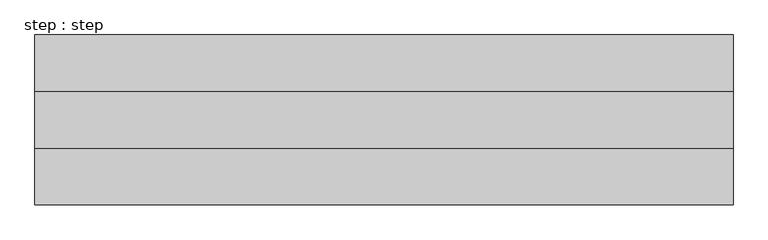
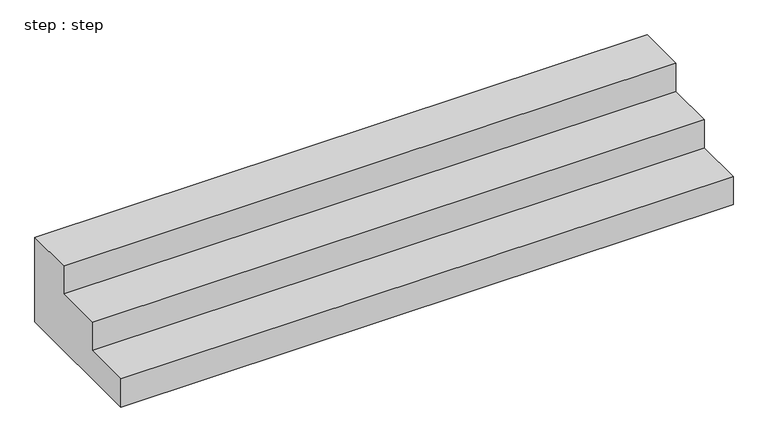
"""IFC4 building model written with IfcOpenShell, lengths in millimetres: proxy geometry, step : step."""

from ifc_helpers import new_model, si_unit, frame, origin, place, context, project, spatial, polyline, outline, extrude, source, transform, mapped, element, save


def step_step_1a2821ed(model_context):
    return source(origin(), model_context, "Body", "SweptSolid", [
        extrude(outline(polyline([(-3204.9933886, 450.0), (-2954.9933886, 450.0), (-2954.9933886, 0.0), (-3704.9933886, 0.0), (-3704.9933886, 150.0), (-3454.9933886, 150.0), (-3454.9933886, 300.0), (-3204.9933886, 300.0), (-3204.9933886, 450.0)])), frame((-15676.5903863, 0.0, 0.0), z_axis=(1.0, 0.0, 0.0), x_axis=(0.0, 1.0, 0.0)), (0.0, 0.0, 1.0), 3085.0),
    ])


if __name__ == "__main__":
    model = new_model("IFC4")
    model_context = context("Model", 3, world=origin())
    ifc_project = project(units=[si_unit("LENGTHUNIT", "METRE", prefix="MILLI")], contexts=[model_context])
    site = spatial("IfcSite", under=ifc_project)
    building = spatial("IfcBuilding", under=site)
    placement = place(None, origin())
    step_step_shape = step_step_1a2821ed(model_context)
    element("IfcBuildingElementProxy", 1, Name="step : step", ObjectType="step : step", at=placement, inside=building, context=model_context, shape_type="MappedRepresentation", body=[
        mapped(step_step_shape, transform((0.0, 0.0, 0.0), x_axis=(1.0, 0.0, 0.0), y_axis=(0.0, 1.0, 0.0), z_axis=(0.0, 0.0, 1.0))),
    ])
    save(model, "model.ifc")
